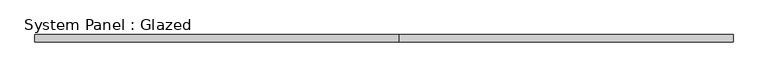
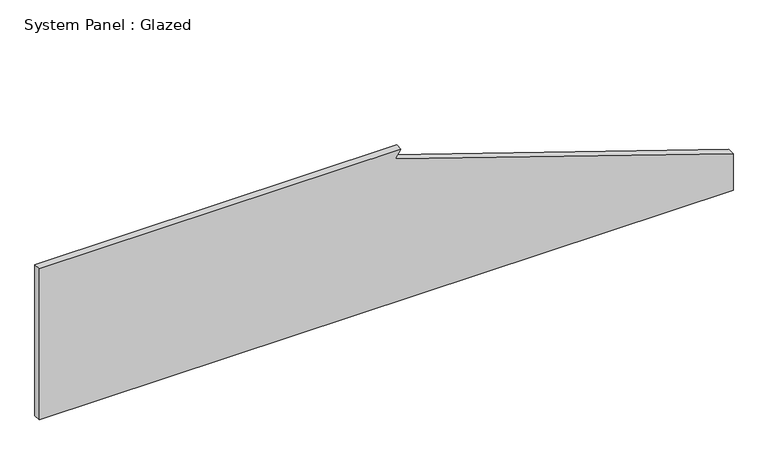
"""IFC4 building model written with IfcOpenShell, lengths in millimetres: plate geometry, System Panel : Glazed."""

from ifc_helpers import new_model, si_unit, frame, origin, place, context, project, spatial, polyline, outline, extrude, source, transform, mapped, element, save


def system_panel_glazed_dff65941(model_context):
    return source(origin(), model_context, "Body", "SweptSolid", [
        extrude(outline(polyline([(0.0, -1187.45), (0.0, 1187.45), (132.0317895, 1187.45), (517.6086106, 30.7195369), (546.1, 50.8), (546.1, -1187.45), (0.0, -1187.45)])), frame((0.0, -44.45, 0.0), z_axis=(0.0, 1.0, 0.0), x_axis=(0.0, 0.0, 1.0)), (0.0, 0.0, 1.0), 25.4),
    ])


if __name__ == "__main__":
    model = new_model("IFC4")
    model_context = context("Model", 3, world=origin())
    ifc_project = project(units=[si_unit("LENGTHUNIT", "METRE", prefix="MILLI")], contexts=[model_context])
    site = spatial("IfcSite", under=ifc_project)
    building = spatial("IfcBuilding", under=site)
    placement = place(None, origin())
    system_panel_glazed_shape = system_panel_glazed_dff65941(model_context)
    element("IfcPlate", 1, ObjectType="System Panel : Glazed", at=placement, inside=building, context=model_context, shape_type="MappedRepresentation", body=[
        mapped(system_panel_glazed_shape, transform((0.0, 0.0, 0.0), x_axis=(1.0, 0.0, 0.0), y_axis=(0.0, 1.0, 0.0), z_axis=(0.0, 0.0, 1.0))),
    ])
    save(model, "model.ifc")

# Revit data of these elements
# Element 1 (IfcPlate, "System Panel : Glazed")
#   Materials on its faces: "Glass"
# Materials
#   "Glass": class "Glass", colour RGB 0 128 192, transparency 0.75
